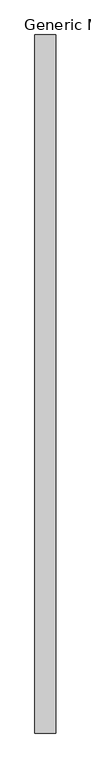
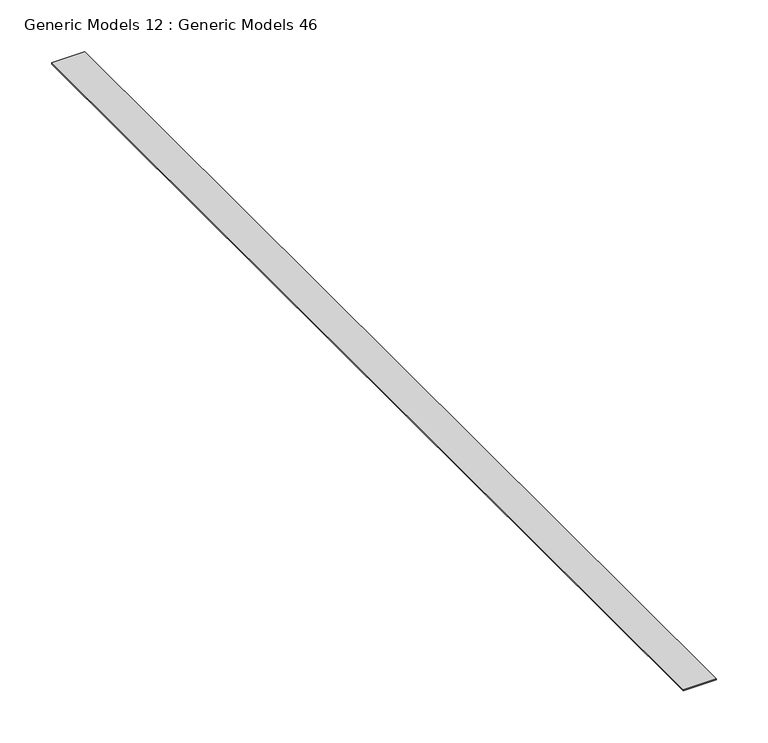
"""IFC4 building model written with IfcOpenShell, lengths in millimetres: proxy geometry, Generic Models 12 : Generic Models 46."""

from ifc_helpers import new_model, si_unit, frame, origin, place, context, project, spatial, polyline, outline, extrude, source, transform, mapped, element, save


def generic_models_12_generic_models_46_b8a9a4e8(model_context):
    return source(origin(), model_context, "Body", "SweptSolid", [
        extrude(outline(polyline([(49757.8505137, 0.0), (49721.1284797, 0.0), (49721.1284797, 1219.2), (49757.8505137, 1219.2), (49757.8505137, 0.0)])), frame((0.0, 0.0, 5505.7509163), z_axis=(0.0, 0.0, 1.0), x_axis=(1.0, 0.0, 0.0)), (0.0, 0.0, 1.0), 1.5875),
    ])


if __name__ == "__main__":
    model = new_model("IFC4")
    model_context = context("Model", 3, world=origin())
    ifc_project = project(units=[si_unit("LENGTHUNIT", "METRE", prefix="MILLI")], contexts=[model_context])
    site = spatial("IfcSite", under=ifc_project)
    building = spatial("IfcBuilding", under=site)
    placement = place(None, origin())
    generic_models_12_generic_models_46_shape = generic_models_12_generic_models_46_b8a9a4e8(model_context)
    element("IfcBuildingElementProxy", 1, Name="Generic Models 12 : Generic Models 46", ObjectType="Generic Models 12 : Generic Models 46", at=placement, inside=building, context=model_context, shape_type="MappedRepresentation", body=[
        mapped(generic_models_12_generic_models_46_shape, transform((0.0, 0.0, 0.0), x_axis=(1.0, 0.0, 0.0), y_axis=(0.0, 1.0, 0.0), z_axis=(0.0, 0.0, 1.0))),
    ])
    save(model, "model.ifc")

# Revit data of these elements
# Element 1 (IfcBuildingElementProxy, "Generic Models 12 : Generic Models 46")
#   Materials on its faces: "SET IN BED OF SEALANT"
# Materials
#   "SET IN BED OF SEALANT": class "Unassigned", colour RGB 58 208 21, transparency 0, Cost = 0
